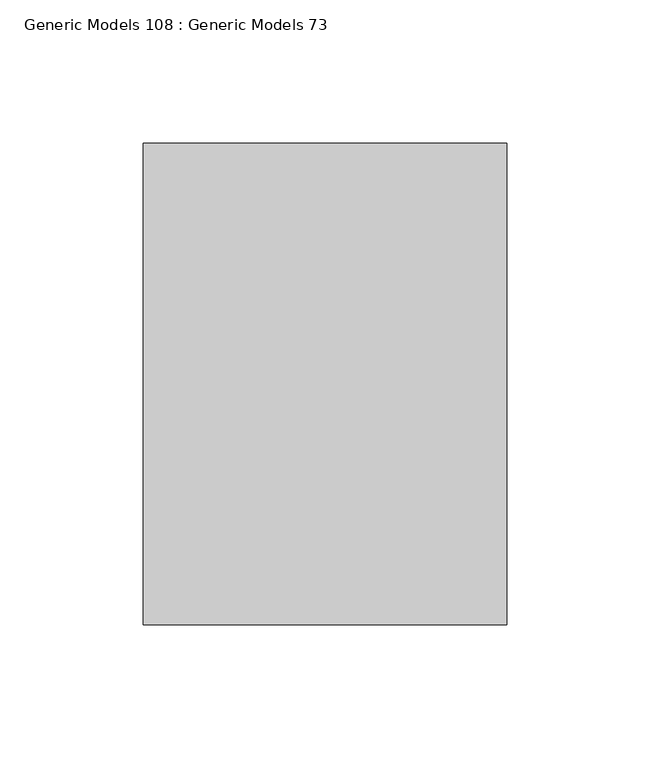
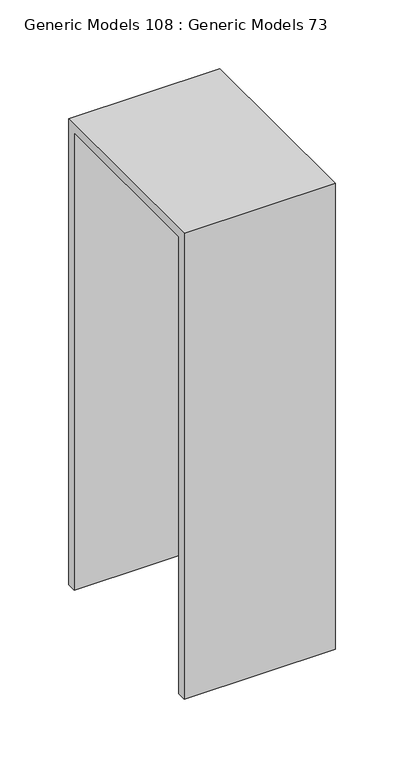
"""IFC4 building model written with IfcOpenShell, lengths in millimetres: proxy geometry, Generic Models 108 : Generic Models 73."""

from ifc_helpers import new_model, si_unit, frame, origin, place, context, project, spatial, polyline, outline, extrude, source, transform, mapped, element, save


def generic_models_108_generic_models_73_f9342414(model_context):
    return source(origin(), model_context, "Body", "SweptSolid", [
        extrude(outline(polyline([(30850.5406612, 271789.525), (30698.1406612, 271789.525), (30698.1406612, 271383.125), (30690.2031612, 271383.125), (30690.2031612, 271797.4625), (30858.4781612, 271797.4625), (30858.4781612, 271383.125), (30850.5406612, 271383.125), (30850.5406612, 271789.525)])), frame((31923.0340778, 0.0, 0.0), z_axis=(1.0, 0.0, 0.0), x_axis=(0.0, 1.0, 0.0)), (0.0, 0.0, 1.0), 127.0),
    ])


if __name__ == "__main__":
    model = new_model("IFC4")
    model_context = context("Model", 3, world=origin())
    ifc_project = project(units=[si_unit("LENGTHUNIT", "METRE", prefix="MILLI")], contexts=[model_context])
    site = spatial("IfcSite", under=ifc_project)
    building = spatial("IfcBuilding", under=site)
    placement = place(None, origin())
    generic_models_108_generic_models_73_shape = generic_models_108_generic_models_73_f9342414(model_context)
    element("IfcBuildingElementProxy", 1, Name="Generic Models 108 : Generic Models 73", ObjectType="Generic Models 108 : Generic Models 73", at=placement, inside=building, context=model_context, shape_type="MappedRepresentation", body=[
        mapped(generic_models_108_generic_models_73_shape, transform((0.0, 0.0, 0.0), x_axis=(1.0, 0.0, 0.0), y_axis=(0.0, 1.0, 0.0), z_axis=(0.0, 0.0, 1.0))),
    ])
    save(model, "model.ifc")

# Revit data of these elements
# Element 1 (IfcBuildingElementProxy, "Generic Models 108 : Generic Models 73")
#   Materials on its faces: "5/16 GALV. PLATE"
# Materials
#   "5/16 GALV. PLATE": class "Metal", colour RGB 199 199 199, transparency 0, Description = "Carbon steel", Cost = 0
